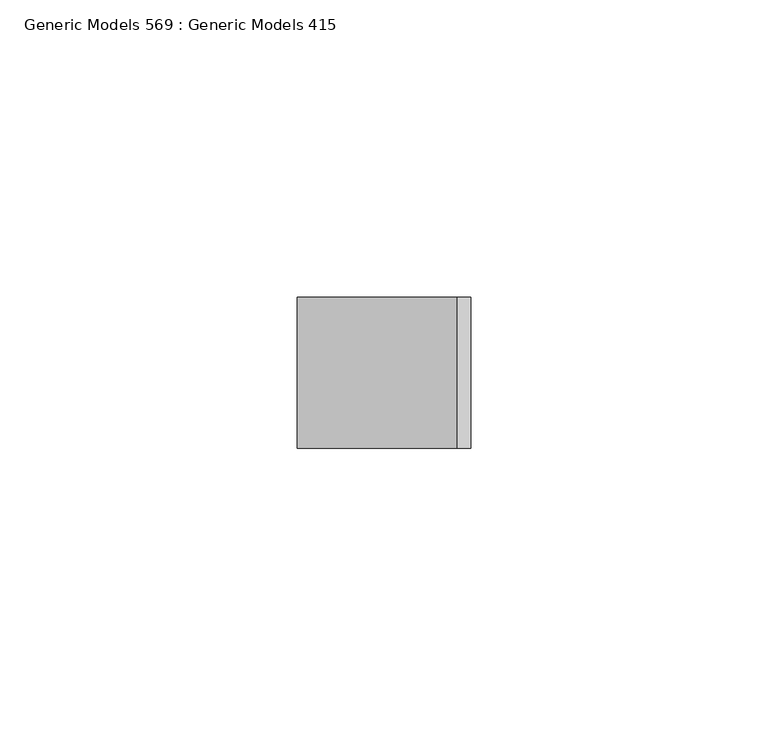
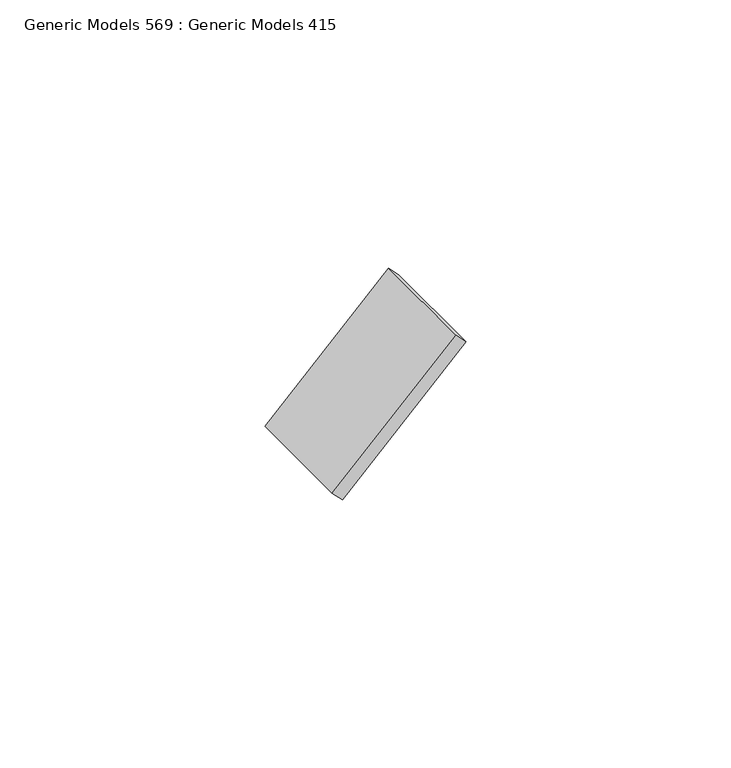
"""IFC4 building model written with IfcOpenShell, lengths in millimetres: proxy geometry, Generic Models 569 : Generic Models 415."""

from ifc_helpers import new_model, si_unit, frame, origin, place, context, project, spatial, polyline, outline, extrude, source, transform, mapped, element, save


def generic_models_569_generic_models_415_6c3201d6(model_context):
    return source(origin(), model_context, "Body", "SweptSolid", [
        extrude(outline(polyline([(0.0, -3.175), (0.0, 0.0), (25.4, 0.0), (25.4, -3.175), (0.0, -3.175)])), frame((7848.0411784, 4501.3863946, 124114.8849742), z_axis=(0.7071067811867181, 0.0, 0.707106781186377), x_axis=(0.0, -1.0, 0.0)), (0.0, 0.0, 1.0), 38.1),
    ])


if __name__ == "__main__":
    model = new_model("IFC4")
    model_context = context("Model", 3, world=origin())
    ifc_project = project(units=[si_unit("LENGTHUNIT", "METRE", prefix="MILLI")], contexts=[model_context])
    site = spatial("IfcSite", under=ifc_project)
    building = spatial("IfcBuilding", under=site)
    placement = place(None, origin())
    generic_models_569_generic_models_415_shape = generic_models_569_generic_models_415_6c3201d6(model_context)
    element("IfcBuildingElementProxy", 1, Name="Generic Models 569 : Generic Models 415", ObjectType="Generic Models 569 : Generic Models 415", at=placement, inside=building, context=model_context, shape_type="MappedRepresentation", body=[
        mapped(generic_models_569_generic_models_415_shape, transform((0.0, 0.0, 0.0), x_axis=(1.0, 0.0, 0.0), y_axis=(0.0, 1.0, 0.0), z_axis=(0.0, 0.0, 1.0))),
    ])
    save(model, "model.ifc")

# Revit data of these elements
# Element 1 (IfcBuildingElementProxy, "Generic Models 569 : Generic Models 415")
#   Materials on its faces: "_WELDED STEEL TABS FOR LOUVER ATTACHMENT"
# Materials
#   "_WELDED STEEL TABS FOR LOUVER ATTACHMENT": class "Metal", colour RGB 199 199 199, transparency 0, Description = "Structural steel 50ksi", Cost = 0
